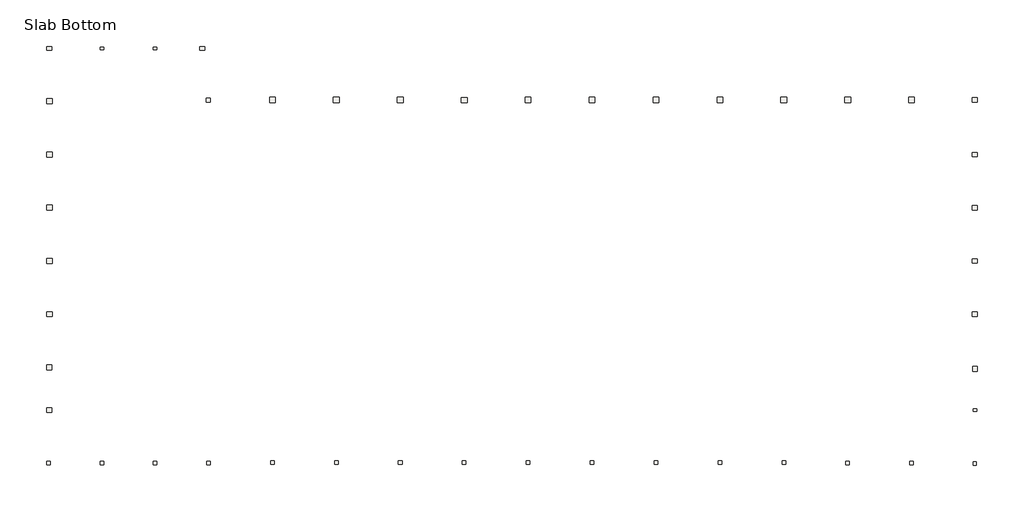
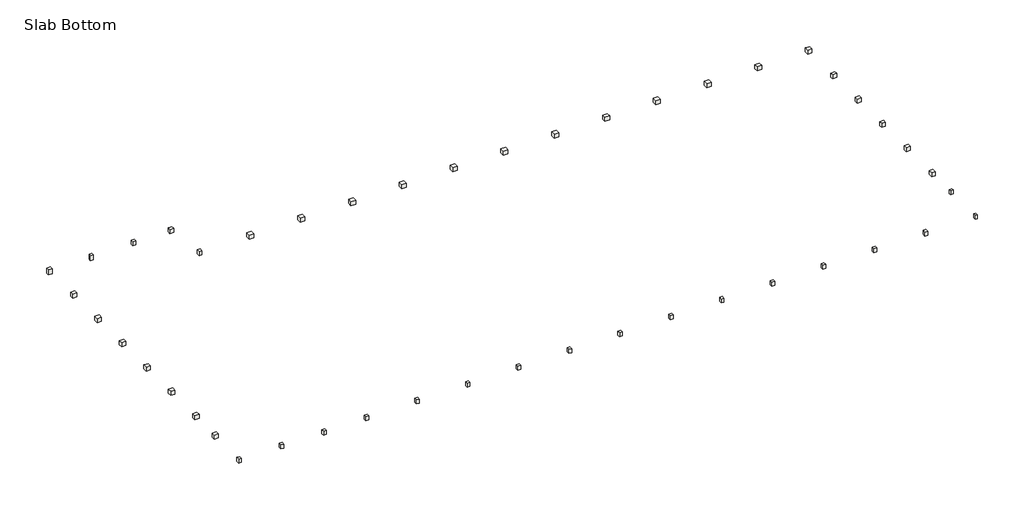
# One storey: 46 slabs.
"""IFC4 building model written with IfcOpenShell, lengths in millimetres."""

from ifc_helpers import new_model, si_unit, frame, origin, place, context, project, spatial, polyline, outline, extrude, faceted_brep, element, save

model = new_model("IFC4")

# Units and contexts
model_context = context("Model", 3, world=origin())
ifc_project = project(units=[si_unit("LENGTHUNIT", "METRE", prefix="MILLI")], contexts=[model_context])

# Site, building, storey
site = spatial("IfcSite", under=ifc_project)
building = spatial("IfcBuilding", under=site)
storey = spatial("IfcBuildingStorey", under=building, Name="Slab Bottom", Elevation=-152.4)

# Slabs
placement = place(None, origin())
element("IfcSlab", 1, ObjectType="Footing-Rectangular : P1", at=placement, inside=storey, context=model_context, shape_type="SweptSolid", body=[
    extrude(outline(polyline([(411246.7398264, -572441.1413841), (411602.3398264, -572441.1413841), (411602.3398264, -572745.9413841), (411246.7398264, -572745.9413841), (411246.7398264, -572441.1413841)])), frame((0.0, 0.0, -914.4), z_axis=(0.0, 0.0, 1.0), x_axis=(1.0, 0.0, 0.0)), (0.0, 0.0, 1.0), 609.6),
])
element("IfcSlab", 2, ObjectType="Footing-Rectangular : P11", at=placement, inside=storey, context=model_context, shape_type="SweptSolid", body=[
    extrude(outline(polyline([(411126.0898264, -549562.0913841), (411126.0898264, -549054.0913841), (411684.8898264, -549054.0913841), (411684.8898264, -549562.0913841), (411126.0898264, -549562.0913841)])), frame((0.0, 0.0, -914.4), z_axis=(0.0, 0.0, 1.0), x_axis=(1.0, 0.0, 0.0)), (0.0, 0.0, 1.0), 609.6),
])
element("IfcSlab", 3, ObjectType="Footing-Rectangular : P11A", at=placement, inside=storey, context=model_context, shape_type="SweptSolid", body=[
    extrude(outline(polyline([(411126.0898264, -561817.5913841), (411126.0898264, -561309.5913841), (411684.8898264, -561309.5913841), (411684.8898264, -561817.5913841), (411126.0898264, -561817.5913841)])), frame((0.0, 0.0, -914.4), z_axis=(0.0, 0.0, 1.0), x_axis=(1.0, 0.0, 0.0)), (0.0, 0.0, 1.0), 609.6),
])
element("IfcSlab", 4, ObjectType="Footing-Rectangular : P12", at=placement, inside=storey, context=model_context, shape_type="SweptSolid", body=[
    extrude(outline(polyline([(304649.2898264, -537331.9913841), (304649.2898264, -536773.1913841), (305258.8898264, -536773.1913841), (305258.8898264, -537331.9913841), (304649.2898264, -537331.9913841)])), frame((0.0, 0.0, -914.4), z_axis=(0.0, 0.0, 1.0), x_axis=(1.0, 0.0, 0.0)), (0.0, 0.0, 1.0), 609.6),
])
element("IfcSlab", 5, ObjectType="Footing-Rectangular : P12", at=placement, inside=storey, context=model_context, shape_type="SweptSolid", body=[
    extrude(outline(polyline([(304649.2898264, -543459.7413841), (304649.2898264, -542900.9413841), (305258.8898264, -542900.9413841), (305258.8898264, -543459.7413841), (304649.2898264, -543459.7413841)])), frame((0.0, 0.0, -914.4), z_axis=(0.0, 0.0, 1.0), x_axis=(1.0, 0.0, 0.0)), (0.0, 0.0, 1.0), 609.6),
])
element("IfcSlab", 6, ObjectType="Footing-Rectangular : P12", at=placement, inside=storey, context=model_context, shape_type="SweptSolid", body=[
    extrude(outline(polyline([(304649.2898264, -549587.4913841), (304649.2898264, -549028.6913841), (305258.8898264, -549028.6913841), (305258.8898264, -549587.4913841), (304649.2898264, -549587.4913841)])), frame((0.0, 0.0, -914.4), z_axis=(0.0, 0.0, 1.0), x_axis=(1.0, 0.0, 0.0)), (0.0, 0.0, 1.0), 609.6),
])
element("IfcSlab", 7, ObjectType="Footing-Rectangular : P12", at=placement, inside=storey, context=model_context, shape_type="SweptSolid", body=[
    extrude(outline(polyline([(304649.2898264, -555715.2413841), (304649.2898264, -555156.4413841), (305258.8898264, -555156.4413841), (305258.8898264, -555715.2413841), (304649.2898264, -555715.2413841)])), frame((0.0, 0.0, -914.4), z_axis=(0.0, 0.0, 1.0), x_axis=(1.0, 0.0, 0.0)), (0.0, 0.0, 1.0), 609.6),
])
element("IfcSlab", 8, ObjectType="Footing-Rectangular : P12", at=placement, inside=storey, context=model_context, shape_type="SweptSolid", body=[
    extrude(outline(polyline([(304649.2898264, -561842.9913841), (304649.2898264, -561284.1913841), (305258.8898264, -561284.1913841), (305258.8898264, -561842.9913841), (304649.2898264, -561842.9913841)])), frame((0.0, 0.0, -914.4), z_axis=(0.0, 0.0, 1.0), x_axis=(1.0, 0.0, 0.0)), (0.0, 0.0, 1.0), 609.6),
])
element("IfcSlab", 9, ObjectType="Footing-Rectangular : P12", at=placement, inside=storey, context=model_context, shape_type="SweptSolid", body=[
    extrude(outline(polyline([(304623.8898264, -567970.7413841), (304623.8898264, -567411.9413841), (305233.4898264, -567411.9413841), (305233.4898264, -567970.7413841), (304623.8898264, -567970.7413841)])), frame((0.0, 0.0, -914.4), z_axis=(0.0, 0.0, 1.0), x_axis=(1.0, 0.0, 0.0)), (0.0, 0.0, 1.0), 609.6),
])
element("IfcSlab", 10, ObjectType="Footing-Rectangular : P13", at=placement, inside=storey, context=model_context, shape_type="SweptSolid", body=[
    extrude(outline(polyline([(403777.974756, -536594.2315281), (404438.374756, -536594.2315281), (404438.374756, -537203.8315281), (403777.974756, -537203.8315281), (403777.974756, -536594.2315281)])), frame((0.0, 0.0, -914.4), z_axis=(0.0, 0.0, 1.0), x_axis=(1.0, 0.0, 0.0)), (0.0, 0.0, 1.0), 609.6),
])
element("IfcSlab", 11, ObjectType="Footing-Rectangular : P13", at=placement, inside=storey, context=model_context, shape_type="SweptSolid", body=[
    extrude(outline(polyline([(396451.2398264, -536601.7413358), (397111.6398264, -536601.7413358), (397111.6398264, -537211.3413358), (396451.2398264, -537211.3413358), (396451.2398264, -536601.7413358)])), frame((0.0, 0.0, -914.4), z_axis=(0.0, 0.0, 1.0), x_axis=(1.0, 0.0, 0.0)), (0.0, 0.0, 1.0), 609.6),
])
element("IfcSlab", 12, ObjectType="Footing-Rectangular : P13", at=placement, inside=storey, context=model_context, shape_type="SweptSolid", body=[
    extrude(outline(polyline([(389097.9398264, -536601.7413358), (389758.3398264, -536601.7413358), (389758.3398264, -537211.3413358), (389097.9398264, -537211.3413358), (389097.9398264, -536601.7413358)])), frame((0.0, 0.0, -914.4), z_axis=(0.0, 0.0, 1.0), x_axis=(1.0, 0.0, 0.0)), (0.0, 0.0, 1.0), 609.6),
])
element("IfcSlab", 13, ObjectType="Footing-Rectangular : P13", at=placement, inside=storey, context=model_context, shape_type="SweptSolid", body=[
    extrude(outline(polyline([(381744.6398264, -536601.7413358), (382405.0398264, -536601.7413358), (382405.0398264, -537211.3413358), (381744.6398264, -537211.3413358), (381744.6398264, -536601.7413358)])), frame((0.0, 0.0, -914.4), z_axis=(0.0, 0.0, 1.0), x_axis=(1.0, 0.0, 0.0)), (0.0, 0.0, 1.0), 609.6),
])
element("IfcSlab", 14, ObjectType="Footing-Rectangular : P13", at=placement, inside=storey, context=model_context, shape_type="SweptSolid", body=[
    extrude(outline(polyline([(374391.3398264, -536601.7413358), (375051.7398264, -536601.7413358), (375051.7398264, -537211.3413358), (374391.3398264, -537211.3413358), (374391.3398264, -536601.7413358)])), frame((0.0, 0.0, -914.4), z_axis=(0.0, 0.0, 1.0), x_axis=(1.0, 0.0, 0.0)), (0.0, 0.0, 1.0), 609.6),
])
element("IfcSlab", 15, ObjectType="Footing-Rectangular : P13", at=placement, inside=storey, context=model_context, shape_type="SweptSolid", body=[
    extrude(outline(polyline([(367038.0398264, -536601.7413358), (367698.4398264, -536601.7413358), (367698.4398264, -537211.3413358), (367038.0398264, -537211.3413358), (367038.0398264, -536601.7413358)])), frame((0.0, 0.0, -914.4), z_axis=(0.0, 0.0, 1.0), x_axis=(1.0, 0.0, 0.0)), (0.0, 0.0, 1.0), 609.6),
])
element("IfcSlab", 16, ObjectType="Footing-Rectangular : P13", at=placement, inside=storey, context=model_context, shape_type="SweptSolid", body=[
    extrude(outline(polyline([(359684.7398264, -536601.7413358), (360345.1398264, -536601.7413358), (360345.1398264, -537211.3413358), (359684.7398264, -537211.3413358), (359684.7398264, -536601.7413358)])), frame((0.0, 0.0, -914.4), z_axis=(0.0, 0.0, 1.0), x_axis=(1.0, 0.0, 0.0)), (0.0, 0.0, 1.0), 609.6),
])
element("IfcSlab", 17, ObjectType="Footing-Rectangular : P13", at=placement, inside=storey, context=model_context, shape_type="SweptSolid", body=[
    extrude(outline(polyline([(352331.4398264, -536614.4413358), (352991.8398264, -536614.4413358), (352991.8398264, -537224.0413358), (352331.4398264, -537224.0413358), (352331.4398264, -536614.4413358)])), frame((0.0, 0.0, -914.4), z_axis=(0.0, 0.0, 1.0), x_axis=(1.0, 0.0, 0.0)), (0.0, 0.0, 1.0), 609.6),
])
element("IfcSlab", 18, ObjectType="Footing-Rectangular : P13", at=placement, inside=storey, context=model_context, shape_type="SweptSolid", body=[
    extrude(outline(polyline([(344978.1398264, -536601.7413358), (345638.5398264, -536601.7413358), (345638.5398264, -537211.3413358), (344978.1398264, -537211.3413358), (344978.1398264, -536601.7413358)])), frame((0.0, 0.0, -914.4), z_axis=(0.0, 0.0, 1.0), x_axis=(1.0, 0.0, 0.0)), (0.0, 0.0, 1.0), 609.6),
])
element("IfcSlab", 19, ObjectType="Footing-Rectangular : P13", at=placement, inside=storey, context=model_context, shape_type="SweptSolid", body=[
    extrude(outline(polyline([(337624.8398264, -536601.7413358), (338285.2398264, -536601.7413358), (338285.2398264, -537211.3413358), (337624.8398264, -537211.3413358), (337624.8398264, -536601.7413358)])), frame((0.0, 0.0, -914.4), z_axis=(0.0, 0.0, 1.0), x_axis=(1.0, 0.0, 0.0)), (0.0, 0.0, 1.0), 609.6),
])
element("IfcSlab", 20, ObjectType="Footing-Rectangular : P13", at=placement, inside=storey, context=model_context, shape_type="SweptSolid", body=[
    extrude(outline(polyline([(330271.5398264, -536601.7413358), (330931.9398264, -536601.7413358), (330931.9398264, -537211.3413358), (330271.5398264, -537211.3413358), (330271.5398264, -536601.7413358)])), frame((0.0, 0.0, -914.4), z_axis=(0.0, 0.0, 1.0), x_axis=(1.0, 0.0, 0.0)), (0.0, 0.0, 1.0), 609.6),
])
element("IfcSlab", 21, ObjectType="Footing-Rectangular : P13A", at=placement, inside=storey, context=model_context, shape_type="SweptSolid", body=[
    extrude(outline(polyline([(411094.3398264, -536620.7913358), (411703.9398264, -536620.7913358), (411703.9398264, -537179.5913358), (411094.3398264, -537179.5913358), (411094.3398264, -536620.7913358)])), frame((0.0, 0.0, -914.4), z_axis=(0.0, 0.0, 1.0), x_axis=(1.0, 0.0, 0.0)), (0.0, 0.0, 1.0), 609.6),
])
element("IfcSlab", 22, ObjectType="Footing-Rectangular : P14", at=placement, inside=storey, context=model_context, shape_type="Brep", body=[
    faceted_brep([(304649.2898264, -572339.5413841, -304.8), (304649.2898264, -572847.5413841, -304.8), (305208.0898264, -572847.5413841, -304.8), (305208.0898264, -572810.8391729, -304.8), (305208.0898264, -572404.4391729, -304.8), (305208.0898264, -572339.5413841, -304.8), (304649.2898264, -572339.5413841, -914.4), (304649.2898264, -572847.5413841, -914.4), (305208.0898264, -572847.5413841, -914.4), (305208.0898264, -572339.5413841, -914.4)], [[[0, 1, 2, 3, 4, 5]], [[1, 0, 6, 7]], [[2, 1, 7, 8]], [[5, 4, 3, 2, 8, 9]], [[0, 5, 9, 6]], [[7, 6, 9, 8]]]),
])
element("IfcSlab", 23, ObjectType="Footing-Rectangular : P2", at=placement, inside=storey, context=model_context, shape_type="SweptSolid", body=[
    extrude(outline(polyline([(322797.5898264, -530747.0413841), (322797.5898264, -531153.4413841), (322238.7898264, -531153.4413841), (322238.7898264, -530747.0413841), (322797.5898264, -530747.0413841)])), frame((0.0, 0.0, -914.4), z_axis=(0.0, 0.0, 1.0), x_axis=(1.0, 0.0, 0.0)), (0.0, 0.0, 1.0), 609.6),
])
element("IfcSlab", 24, ObjectType="Footing-Rectangular : P3", at=placement, inside=storey, context=model_context, shape_type="SweptSolid", body=[
    extrude(outline(polyline([(411246.7398264, -578543.4913841), (411551.5398264, -578543.4913841), (411551.5398264, -578949.8913841), (411246.7398264, -578949.8913841), (411246.7398264, -578543.4913841)])), frame((0.0, 0.0, -914.4), z_axis=(0.0, 0.0, 1.0), x_axis=(1.0, 0.0, 0.0)), (0.0, 0.0, 1.0), 609.6),
])
element("IfcSlab", 25, ObjectType="Footing-Rectangular : P4", at=placement, inside=storey, context=model_context, shape_type="SweptSolid", body=[
    extrude(outline(polyline([(310789.7398264, -531108.9913841), (310789.7398264, -530804.1913841), (311196.1398264, -530804.1913841), (311196.1398264, -531108.9913841), (310789.7398264, -531108.9913841)])), frame((0.0, 0.0, -1066.8), z_axis=(0.0, 0.0, 1.0), x_axis=(1.0, 0.0, 0.0)), (0.0, 0.0, 1.0), 762.0),
])
element("IfcSlab", 26, ObjectType="Footing-Rectangular : P4", at=placement, inside=storey, context=model_context, shape_type="SweptSolid", body=[
    extrude(outline(polyline([(317323.8898264, -531108.9913841), (316917.4898264, -531108.9913841), (316917.4898264, -530804.1913841), (317323.8898264, -530804.1913841), (317323.8898264, -531108.9913841)])), frame((0.0, 0.0, -914.4), z_axis=(0.0, 0.0, 1.0), x_axis=(1.0, 0.0, 0.0)), (0.0, 0.0, 1.0), 609.6),
])
element("IfcSlab", 27, ObjectType="Footing-Rectangular : P5", at=placement, inside=storey, context=model_context, shape_type="SweptSolid", body=[
    extrude(outline(polyline([(311196.1398264, -578892.7413841), (310789.7398264, -578892.7413841), (310789.7398264, -578486.3413841), (311196.1398264, -578486.3413841), (311196.1398264, -578892.7413841)])), frame((0.0, 0.0, -914.4), z_axis=(0.0, 0.0, 1.0), x_axis=(1.0, 0.0, 0.0)), (0.0, 0.0, 1.0), 609.6),
])
element("IfcSlab", 28, ObjectType="Footing-Rectangular : P5", at=placement, inside=storey, context=model_context, shape_type="SweptSolid", body=[
    extrude(outline(polyline([(317327.0648264, -578937.1913841), (316920.6648264, -578937.1913841), (316920.6648264, -578530.7913841), (317327.0648264, -578530.7913841), (317327.0648264, -578937.1913841)])), frame((0.0, 0.0, -914.4), z_axis=(0.0, 0.0, 1.0), x_axis=(1.0, 0.0, 0.0)), (0.0, 0.0, 1.0), 609.6),
])
element("IfcSlab", 29, ObjectType="Footing-Rectangular : P5", at=placement, inside=storey, context=model_context, shape_type="SweptSolid", body=[
    extrude(outline(polyline([(330398.5398264, -578448.2413841), (330804.9398264, -578448.2413841), (330804.9398264, -578854.6413841), (330398.5398264, -578854.6413841), (330398.5398264, -578448.2413841)])), frame((0.0, 0.0, -914.4), z_axis=(0.0, 0.0, 1.0), x_axis=(1.0, 0.0, 0.0)), (0.0, 0.0, 1.0), 609.6),
])
element("IfcSlab", 30, ObjectType="Footing-Rectangular : P5", at=placement, inside=storey, context=model_context, shape_type="SweptSolid", body=[
    extrude(outline(polyline([(337751.8398264, -578448.2413841), (338158.2398264, -578448.2413841), (338158.2398264, -578854.6413841), (337751.8398264, -578854.6413841), (337751.8398264, -578448.2413841)])), frame((0.0, 0.0, -914.4), z_axis=(0.0, 0.0, 1.0), x_axis=(1.0, 0.0, 0.0)), (0.0, 0.0, 1.0), 609.6),
])
element("IfcSlab", 31, ObjectType="Footing-Rectangular : P5", at=placement, inside=storey, context=model_context, shape_type="SweptSolid", body=[
    extrude(outline(polyline([(345105.1398264, -578448.2413841), (345511.5398264, -578448.2413841), (345511.5398264, -578854.6413841), (345105.1398264, -578854.6413841), (345105.1398264, -578448.2413841)])), frame((0.0, 0.0, -914.4), z_axis=(0.0, 0.0, 1.0), x_axis=(1.0, 0.0, 0.0)), (0.0, 0.0, 1.0), 609.6),
])
element("IfcSlab", 32, ObjectType="Footing-Rectangular : P5", at=placement, inside=storey, context=model_context, shape_type="SweptSolid", body=[
    extrude(outline(polyline([(352458.4398264, -578448.2413841), (352864.8398264, -578448.2413841), (352864.8398264, -578854.6413841), (352458.4398264, -578854.6413841), (352458.4398264, -578448.2413841)])), frame((0.0, 0.0, -914.4), z_axis=(0.0, 0.0, 1.0), x_axis=(1.0, 0.0, 0.0)), (0.0, 0.0, 1.0), 609.6),
])
element("IfcSlab", 33, ObjectType="Footing-Rectangular : P5", at=placement, inside=storey, context=model_context, shape_type="SweptSolid", body=[
    extrude(outline(polyline([(359811.7398264, -578448.2413841), (360218.1398264, -578448.2413841), (360218.1398264, -578854.6413841), (359811.7398264, -578854.6413841), (359811.7398264, -578448.2413841)])), frame((0.0, 0.0, -914.4), z_axis=(0.0, 0.0, 1.0), x_axis=(1.0, 0.0, 0.0)), (0.0, 0.0, 1.0), 609.6),
])
element("IfcSlab", 34, ObjectType="Footing-Rectangular : P5", at=placement, inside=storey, context=model_context, shape_type="SweptSolid", body=[
    extrude(outline(polyline([(367165.0398264, -578448.2413841), (367571.4398264, -578448.2413841), (367571.4398264, -578854.6413841), (367165.0398264, -578854.6413841), (367165.0398264, -578448.2413841)])), frame((0.0, 0.0, -914.4), z_axis=(0.0, 0.0, 1.0), x_axis=(1.0, 0.0, 0.0)), (0.0, 0.0, 1.0), 609.6),
])
element("IfcSlab", 35, ObjectType="Footing-Rectangular : P5", at=placement, inside=storey, context=model_context, shape_type="SweptSolid", body=[
    extrude(outline(polyline([(374518.3398264, -578448.2413841), (374924.7398264, -578448.2413841), (374924.7398264, -578854.6413841), (374518.3398264, -578854.6413841), (374518.3398264, -578448.2413841)])), frame((0.0, 0.0, -914.4), z_axis=(0.0, 0.0, 1.0), x_axis=(1.0, 0.0, 0.0)), (0.0, 0.0, 1.0), 609.6),
])
element("IfcSlab", 36, ObjectType="Footing-Rectangular : P5", at=placement, inside=storey, context=model_context, shape_type="SweptSolid", body=[
    extrude(outline(polyline([(381871.6398264, -578448.2413841), (382278.0398264, -578448.2413841), (382278.0398264, -578854.6413841), (381871.6398264, -578854.6413841), (381871.6398264, -578448.2413841)])), frame((0.0, 0.0, -914.4), z_axis=(0.0, 0.0, 1.0), x_axis=(1.0, 0.0, 0.0)), (0.0, 0.0, 1.0), 609.6),
])
element("IfcSlab", 37, ObjectType="Footing-Rectangular : P5", at=placement, inside=storey, context=model_context, shape_type="SweptSolid", body=[
    extrude(outline(polyline([(389224.9398264, -578448.2413841), (389631.3398264, -578448.2413841), (389631.3398264, -578854.6413841), (389224.9398264, -578854.6413841), (389224.9398264, -578448.2413841)])), frame((0.0, 0.0, -914.4), z_axis=(0.0, 0.0, 1.0), x_axis=(1.0, 0.0, 0.0)), (0.0, 0.0, 1.0), 609.6),
])
element("IfcSlab", 38, ObjectType="Footing-Rectangular : P5", at=placement, inside=storey, context=model_context, shape_type="SweptSolid", body=[
    extrude(outline(polyline([(403931.5398264, -578530.7913841), (404337.9398264, -578530.7913841), (404337.9398264, -578937.1913841), (403931.5398264, -578937.1913841), (403931.5398264, -578530.7913841)])), frame((0.0, 0.0, -914.4), z_axis=(0.0, 0.0, 1.0), x_axis=(1.0, 0.0, 0.0)), (0.0, 0.0, 1.0), 609.6),
])
element("IfcSlab", 39, ObjectType="Footing-Rectangular : P5A", at=placement, inside=storey, context=model_context, shape_type="SweptSolid", body=[
    extrude(outline(polyline([(396578.2398264, -578530.7913841), (396984.6398264, -578530.7913841), (396984.6398264, -578937.1913841), (396578.2398264, -578937.1913841), (396578.2398264, -578530.7913841)])), frame((0.0, 0.0, -914.4), z_axis=(0.0, 0.0, 1.0), x_axis=(1.0, 0.0, 0.0)), (0.0, 0.0, 1.0), 609.6),
])
element("IfcSlab", 40, ObjectType="Footing-Rectangular : P5B", at=placement, inside=storey, context=model_context, shape_type="SweptSolid", body=[
    extrude(outline(polyline([(323064.2898264, -578899.0913841), (323064.2898264, -578492.6913841), (323470.6898264, -578492.6913841), (323470.6898264, -578899.0913841), (323064.2898264, -578899.0913841)])), frame((0.0, 0.0, -914.4), z_axis=(0.0, 0.0, 1.0), x_axis=(1.0, 0.0, 0.0)), (0.0, 0.0, 1.0), 609.6),
])
element("IfcSlab", 41, ObjectType="Footing-Rectangular : P5C", at=placement, inside=storey, context=model_context, shape_type="SweptSolid", body=[
    extrude(outline(polyline([(304642.9398264, -578899.0913841), (304642.9398264, -578492.6913841), (305049.3398264, -578492.6913841), (305049.3398264, -578899.0913841), (304642.9398264, -578899.0913841)])), frame((0.0, 0.0, -914.4), z_axis=(0.0, 0.0, 1.0), x_axis=(1.0, 0.0, 0.0)), (0.0, 0.0, 1.0), 609.6),
])
element("IfcSlab", 42, ObjectType="Footing-Rectangular : P6", at=placement, inside=storey, context=model_context, shape_type="SweptSolid", body=[
    extrude(outline(polyline([(323019.8398264, -536722.3913841), (323426.2398264, -536722.3913841), (323426.2398264, -537179.5913841), (323019.8398264, -537179.5913841), (323019.8398264, -536722.3913841)])), frame((0.0, 0.0, -914.4), z_axis=(0.0, 0.0, 1.0), x_axis=(1.0, 0.0, 0.0)), (0.0, 0.0, 1.0), 609.6),
])
element("IfcSlab", 43, ObjectType="Footing-Rectangular : P6A", at=placement, inside=storey, context=model_context, shape_type="SweptSolid", body=[
    extrude(outline(polyline([(304655.6398264, -530747.0413841), (305214.4398264, -530747.0413841), (305214.4398264, -531153.4413841), (304655.6398264, -531153.4413841), (304655.6398264, -530747.0413841)])), frame((0.0, 0.0, -1066.8), z_axis=(0.0, 0.0, 1.0), x_axis=(1.0, 0.0, 0.0)), (0.0, 0.0, 1.0), 762.0),
])
element("IfcSlab", 44, ObjectType="Footing-Rectangular : P7", at=placement, inside=storey, context=model_context, shape_type="SweptSolid", body=[
    extrude(outline(polyline([(411145.1398264, -567577.0413841), (411653.1398264, -567577.0413841), (411653.1398264, -568135.8413841), (411145.1398264, -568135.8413841), (411145.1398264, -567577.0413841)])), frame((0.0, 0.0, -914.4), z_axis=(0.0, 0.0, 1.0), x_axis=(1.0, 0.0, 0.0)), (0.0, 0.0, 1.0), 609.6),
])
element("IfcSlab", 45, ObjectType="Footing-Rectangular : P8", at=placement, inside=storey, context=model_context, shape_type="SweptSolid", body=[
    extrude(outline(polyline([(411126.0898264, -555664.4413841), (411126.0898264, -555207.2413841), (411684.8898264, -555207.2413841), (411684.8898264, -555664.4413841), (411126.0898264, -555664.4413841)])), frame((0.0, 0.0, -914.4), z_axis=(0.0, 0.0, 1.0), x_axis=(1.0, 0.0, 0.0)), (0.0, 0.0, 1.0), 609.6),
])
element("IfcSlab", 46, ObjectType="Footing-Rectangular : P9", at=placement, inside=storey, context=model_context, shape_type="SweptSolid", body=[
    extrude(outline(polyline([(411094.3398264, -543408.9413841), (411094.3398264, -542951.7413841), (411703.9398264, -542951.7413841), (411703.9398264, -543408.9413841), (411094.3398264, -543408.9413841)])), frame((0.0, 0.0, -914.4), z_axis=(0.0, 0.0, 1.0), x_axis=(1.0, 0.0, 0.0)), (0.0, 0.0, 1.0), 609.6),
])

save(model, "model.ifc")

# Revit data of these elements
# Type "Footing-Rectangular : P1"
#   Type Mark = ""
#   Assembly Code = "A1010100"
#   Width = 1' - 2"
#   Length = 1' - 0"
#   Thickness = 2' - 6"
#   Structural Material [instance default] = CONCRETE FOOTING - SEE STRUCT DWGS.
# Type "Footing-Rectangular : P11"
#   Assembly Code = "A1010100"
#   Width = 1' - 8"
#   Length = 1' - 10"
#   Thickness = 2' - 6"
#   Structural Material [instance default] = CONCRETE FOOTING - SEE STRUCT DWGS.
# Type "Footing-Rectangular : P11A"
#   Assembly Code = "A1010100"
#   Width = 1' - 8"
#   Length = 1' - 10"
#   Thickness = 2' - 6"
#   Structural Material [instance default] = CONCRETE FOOTING - SEE STRUCT DWGS.
# Type "Footing-Rectangular : P12"
#   Assembly Code = "A1010100"
#   Width = 1' - 10"
#   Length = 2' - 0"
#   Thickness = 2' - 6"
#   Structural Material [instance default] = CONCRETE FOOTING - SEE STRUCT DWGS.
# Type "Footing-Rectangular : P13"
#   Assembly Code = "A1010100"
#   Width = 2' - 2"
#   Length = 2' - 0"
#   Thickness = 2' - 6"
#   Structural Material [instance default] = CONCRETE FOOTING - SEE STRUCT DWGS.
# Type "Footing-Rectangular : P13A"
#   Assembly Code = "A1010100"
#   Width = 2' - 0"
#   Length = 1' - 10"
#   Thickness = 2' - 6"
#   Structural Material [instance default] = CONCRETE FOOTING - SEE STRUCT DWGS.
# Type "Footing-Rectangular : P14"
#   Assembly Code = "A1010100"
#   Width = 1' - 8"
#   Length = 1' - 10"
#   Thickness = 2' - 6"
#   Structural Material [instance default] = CONCRETE FOOTING - SEE STRUCT DWGS.
# Type "Footing-Rectangular : P2"
#   Assembly Code = "A1010100"
#   Width = 1' - 4"
#   Length = 1' - 10"
#   Thickness = 2' - 6"
#   Structural Material [instance default] = CONCRETE FOOTING - SEE STRUCT DWGS.
# Type "Footing-Rectangular : P3"
#   Assembly Code = "A1010100"
#   Width = 1' - 0"
#   Length = 1' - 4"
#   Thickness = 2' - 6"
#   Structural Material [instance default] = CONCRETE FOOTING - SEE STRUCT DWGS.
# Type "Footing-Rectangular : P4"
#   Assembly Code = "A1010100"
#   Width = 1' - 4"
#   Length = 1' - 0"
#   Thickness = 2' - 6"
#   Structural Material [instance default] = CONCRETE FOOTING - SEE STRUCT DWGS.
# Type "Footing-Rectangular : P5"
#   Assembly Code = "A1010100"
#   Width = 1' - 4"
#   Length = 1' - 4"
#   Thickness = 2' - 6"
#   Structural Material [instance default] = CONCRETE FOOTING - SEE STRUCT DWGS.
# Type "Footing-Rectangular : P5A"
#   Assembly Code = "A1010100"
#   Width = 1' - 4"
#   Length = 1' - 4"
#   Thickness = 2' - 6"
#   Structural Material [instance default] = CONCRETE FOOTING - SEE STRUCT DWGS.
# Type "Footing-Rectangular : P5B"
#   Assembly Code = "A1010100"
#   Width = 1' - 4"
#   Length = 1' - 4"
#   Thickness = 2' - 6"
#   Structural Material [instance default] = CONCRETE FOOTING - SEE STRUCT DWGS.
# Type "Footing-Rectangular : P5C"
#   Assembly Code = "A1010100"
#   Width = 1' - 4"
#   Length = 1' - 4"
#   Thickness = 2' - 6"
#   Structural Material [instance default] = CONCRETE FOOTING - SEE STRUCT DWGS.
# Type "Footing-Rectangular : P6"
#   Assembly Code = "A1010100"
#   Width = 1' - 4"
#   Length = 1' - 6"
#   Thickness = 2' - 6"
#   Structural Material [instance default] = CONCRETE FOOTING - SEE STRUCT DWGS.
# Type "Footing-Rectangular : P6A"
#   Assembly Code = "A1010100"
#   Width = 1' - 4"
#   Length = 1' - 10"
#   Thickness = 2' - 6"
#   Structural Material [instance default] = CONCRETE FOOTING - SEE STRUCT DWGS.
# Type "Footing-Rectangular : P7"
#   Assembly Code = "A1010100"
#   Width = 1' - 8"
#   Length = 1' - 10"
#   Thickness = 2' - 6"
#   Structural Material [instance default] = CONCRETE FOOTING - SEE STRUCT DWGS.
# Type "Footing-Rectangular : P8"
#   Assembly Code = "A1010100"
#   Width = 1' - 6"
#   Length = 1' - 10"
#   Thickness = 2' - 6"
#   Structural Material [instance default] = CONCRETE FOOTING - SEE STRUCT DWGS.
# Type "Footing-Rectangular : P9"
#   Assembly Code = "A1010100"
#   Width = 1' - 6"
#   Length = 2' - 0"
#   Thickness = 2' - 6"
#   Structural Material [instance default] = CONCRETE FOOTING - SEE STRUCT DWGS.
# Element 1 (IfcSlab, "Footing-Rectangular : P1")
#   Comments = ""
#   Structural Material = CONCRETE PIER- SEE STRUCT DWGS.
#   Phase Created = New Construction
#   Materials on its faces: "CONCRETE PIER- SEE STRUCT DWGS.", "CONCRETE FOOTING - SEE STRUCT DWGS."
# Element 2 (IfcSlab, "Footing-Rectangular : P11")
#   Comments = ""
#   Structural Material = CONCRETE PIER- SEE STRUCT DWGS.
#   Phase Created = New Construction
#   Materials on its faces: "CONCRETE PIER- SEE STRUCT DWGS.", "CONCRETE FOOTING - SEE STRUCT DWGS."
# Element 3 (IfcSlab, "Footing-Rectangular : P11A")
#   Comments = ""
#   Structural Material = CONCRETE PIER- SEE STRUCT DWGS.
#   Phase Created = New Construction
#   Materials on its faces: "CONCRETE PIER- SEE STRUCT DWGS.", "CONCRETE FOOTING - SEE STRUCT DWGS."
# Elements 4, 5, 6, 7, 8, 9 (IfcSlab, "Footing-Rectangular : P12")
#   Comments = ""
#   Structural Material = CONCRETE PIER- SEE STRUCT DWGS.
#   Phase Created = New Construction
#   Materials on its faces: "CONCRETE PIER- SEE STRUCT DWGS.", "CONCRETE FOOTING - SEE STRUCT DWGS."
# Elements 10, 11, 12, 13, 14, 15, 16, 17, 18, 19, 20 (IfcSlab, "Footing-Rectangular : P13")
#   Comments = ""
#   Structural Material = CONCRETE PIER- SEE STRUCT DWGS.
#   Phase Created = New Construction
#   Materials on its faces: "CONCRETE PIER- SEE STRUCT DWGS.", "CONCRETE FOOTING - SEE STRUCT DWGS."
# Element 21 (IfcSlab, "Footing-Rectangular : P13A")
#   Comments = ""
#   Structural Material = CONCRETE PIER- SEE STRUCT DWGS.
#   Phase Created = New Construction
#   Materials on its faces: "CONCRETE PIER- SEE STRUCT DWGS.", "CONCRETE FOOTING - SEE STRUCT DWGS."
# Element 22 (IfcSlab, "Footing-Rectangular : P14")
#   Comments = ""
#   Structural Material = CONCRETE PIER- SEE STRUCT DWGS.
#   Phase Created = New Construction
#   Materials on its faces: "CONCRETE PIER- SEE STRUCT DWGS.", "CONCRETE FOOTING - SEE STRUCT DWGS."
# Element 23 (IfcSlab, "Footing-Rectangular : P2")
#   Comments = ""
#   Structural Material = CONCRETE PIER- SEE STRUCT DWGS.
#   Phase Created = New Construction
#   Materials on its faces: "CONCRETE PIER- SEE STRUCT DWGS.", "CONCRETE FOOTING - SEE STRUCT DWGS."
# Element 24 (IfcSlab, "Footing-Rectangular : P3")
#   Comments = ""
#   Structural Material = CONCRETE PIER- SEE STRUCT DWGS.
#   Phase Created = New Construction
#   Materials on its faces: "CONCRETE PIER- SEE STRUCT DWGS.", "CONCRETE FOOTING - SEE STRUCT DWGS."
# Element 25 (IfcSlab, "Footing-Rectangular : P4")
#   Comments = ""
#   Structural Material = CONCRETE PIER- SEE STRUCT DWGS.
#   Phase Created = New Construction
#   Materials on its faces: "CONCRETE PIER- SEE STRUCT DWGS."
# Element 26 (IfcSlab, "Footing-Rectangular : P4")
#   Comments = ""
#   Structural Material = CONCRETE PIER- SEE STRUCT DWGS.
#   Phase Created = New Construction
#   Materials on its faces: "CONCRETE PIER- SEE STRUCT DWGS.", "CONCRETE FOOTING - SEE STRUCT DWGS."
# Elements 27, 28, 29, 30, 31, 32, 33, 34, 35, 36, 37, 38 (IfcSlab, "Footing-Rectangular : P5")
#   Comments = ""
#   Structural Material = CONCRETE PIER- SEE STRUCT DWGS.
#   Phase Created = New Construction
#   Materials on its faces: "CONCRETE PIER- SEE STRUCT DWGS.", "CONCRETE FOOTING - SEE STRUCT DWGS."
# Element 39 (IfcSlab, "Footing-Rectangular : P5A")
#   Comments = ""
#   Structural Material = CONCRETE PIER- SEE STRUCT DWGS.
#   Phase Created = New Construction
#   Materials on its faces: "CONCRETE PIER- SEE STRUCT DWGS.", "CONCRETE FOOTING - SEE STRUCT DWGS."
# Element 40 (IfcSlab, "Footing-Rectangular : P5B")
#   Comments = ""
#   Structural Material = CONCRETE PIER- SEE STRUCT DWGS.
#   Phase Created = New Construction
#   Materials on its faces: "CONCRETE PIER- SEE STRUCT DWGS.", "CONCRETE FOOTING - SEE STRUCT DWGS."
# Element 41 (IfcSlab, "Footing-Rectangular : P5C")
#   Comments = ""
#   Structural Material = CONCRETE PIER- SEE STRUCT DWGS.
#   Phase Created = New Construction
#   Materials on its faces: "CONCRETE PIER- SEE STRUCT DWGS.", "CONCRETE FOOTING - SEE STRUCT DWGS."
# Element 42 (IfcSlab, "Footing-Rectangular : P6")
#   Comments = ""
#   Structural Material = CONCRETE PIER- SEE STRUCT DWGS.
#   Phase Created = New Construction
#   Materials on its faces: "CONCRETE PIER- SEE STRUCT DWGS.", "CONCRETE FOOTING - SEE STRUCT DWGS."
# Element 43 (IfcSlab, "Footing-Rectangular : P6A")
#   Comments = ""
#   Structural Material = CONCRETE PIER- SEE STRUCT DWGS.
#   Phase Created = New Construction
#   Materials on its faces: "CONCRETE PIER- SEE STRUCT DWGS."
# Element 44 (IfcSlab, "Footing-Rectangular : P7")
#   Comments = ""
#   Structural Material = CONCRETE PIER- SEE STRUCT DWGS.
#   Phase Created = New Construction
#   Materials on its faces: "CONCRETE PIER- SEE STRUCT DWGS.", "CONCRETE FOOTING - SEE STRUCT DWGS."
# Element 45 (IfcSlab, "Footing-Rectangular : P8")
#   Comments = ""
#   Structural Material = CONCRETE PIER- SEE STRUCT DWGS.
#   Phase Created = New Construction
#   Materials on its faces: "CONCRETE PIER- SEE STRUCT DWGS.", "CONCRETE FOOTING - SEE STRUCT DWGS."
# Element 46 (IfcSlab, "Footing-Rectangular : P9")
#   Comments = ""
#   Structural Material = CONCRETE PIER- SEE STRUCT DWGS.
#   Phase Created = New Construction
#   Materials on its faces: "CONCRETE PIER- SEE STRUCT DWGS.", "CONCRETE FOOTING - SEE STRUCT DWGS."
# Materials
#   "CONCRETE FOOTING - SEE STRUCT DWGS.": class "Concrete", colour RGB 192 192 192, transparency 0, Description = "Cast-in-place concrete", Cost = 0
#   "CONCRETE PIER- SEE STRUCT DWGS.": class "Concrete", colour RGB 192 192 192, transparency 0, Description = "Cast-in-place concrete", Cost = 0
